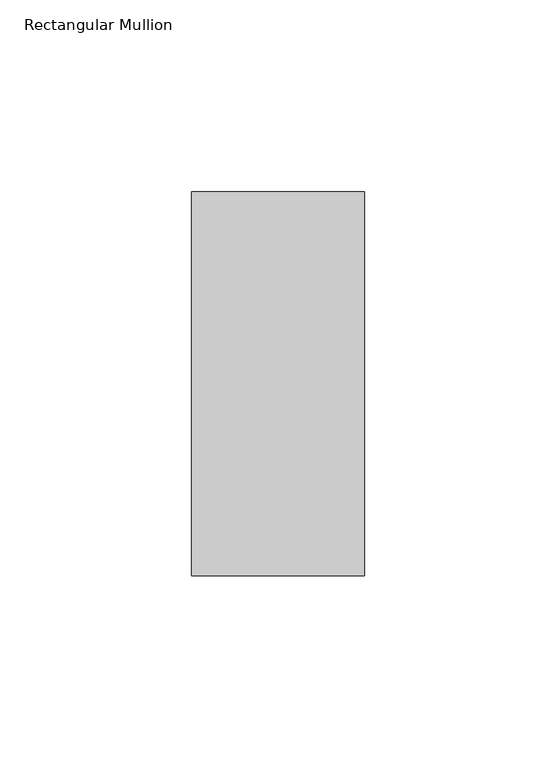
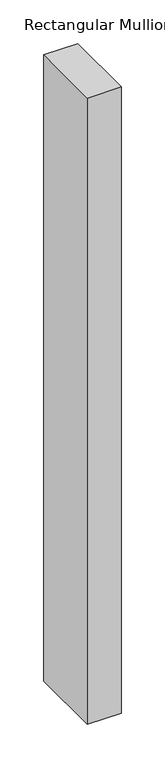
"""IFC4 building model written with IfcOpenShell, lengths in millimetres: member geometry, Rectangular Mullion : 알루미늄_Rectangular Cap_100 x 45."""

from ifc_helpers import new_model, si_unit, frame, origin, place, context, project, spatial, polyline, outline, extrude, source, transform, mapped, element, save


def rectangular_mullion_c63874d8(model_context):
    return source(origin(), model_context, "Body", "SweptSolid", [
        extrude(outline(polyline([(0.0, 50.0), (0.0, -50.0), (-45.0, -50.0), (-45.0, 50.0), (0.0, 50.0)])), frame((0.0, 0.0, -877.5), z_axis=(0.0, 0.0, 1.0), x_axis=(1.0, 0.0, 0.0)), (0.0, 0.0, 1.0), 877.5),
    ])


if __name__ == "__main__":
    model = new_model("IFC4")
    model_context = context("Model", 3, world=origin())
    ifc_project = project(units=[si_unit("LENGTHUNIT", "METRE", prefix="MILLI")], contexts=[model_context])
    site = spatial("IfcSite", under=ifc_project)
    building = spatial("IfcBuilding", under=site)
    placement = place(None, origin())
    rectangular_mullion_shape = rectangular_mullion_c63874d8(model_context)
    element("IfcMember", 1, ObjectType="Rectangular Mullion : 알루미늄_Rectangular Cap_100 x 45", at=placement, inside=building, context=model_context, shape_type="MappedRepresentation", body=[
        mapped(rectangular_mullion_shape, transform((0.0, 0.0, 0.0), x_axis=(1.0, 0.0, 0.0), y_axis=(0.0, 1.0, 0.0), z_axis=(0.0, 0.0, 1.0))),
    ])
    save(model, "model.ifc")

# Revit data of these elements
# Type "Rectangular Mullion : 알루미늄_Rectangular Cap_100 x 45"
#   built-in parameter 1007304 = 0.328084 (stored number, unit not read)
#   built-in parameter 1007301 = 0.0738189 (stored number, unit not read)
#   built-in parameter 1007300 = 0.0738189 (stored number, unit not read)
# Element 1 (IfcMember, "Rectangular Mullion : 알루미늄_Rectangular Cap_100 x 45")
#   Materials on its faces: "00_Metal_Stainless Steel"
# Materials
#   "00_Metal_Stainless Steel": class "Metal", colour RGB 148 148 148, transparency 0, Description = "Steel", Cost = 0
